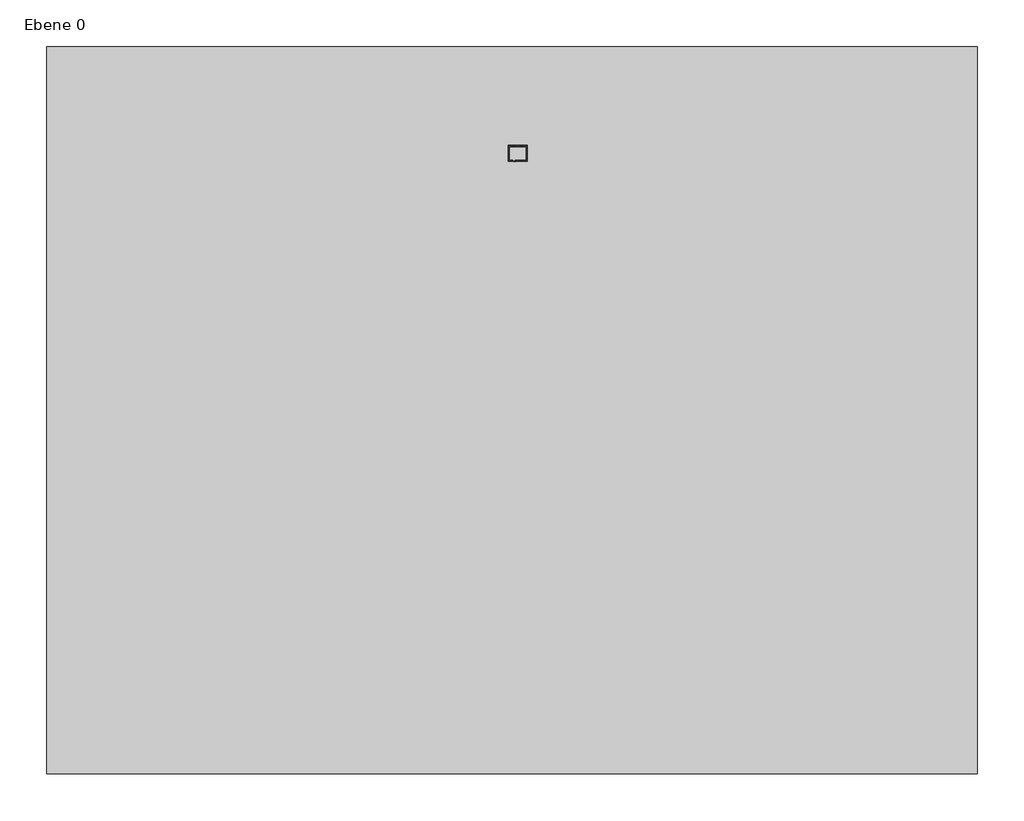
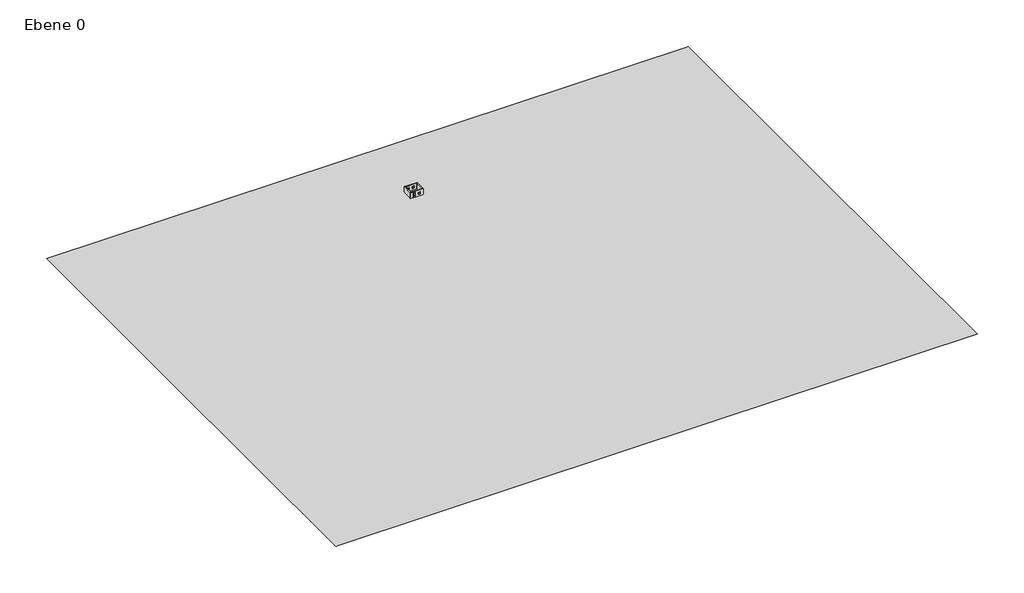
# One storey: 4 walls, 3 windows, 2 proxies, 1 door.
"""IFC4 building model written with IfcOpenShell, lengths in millimetres."""

import ifcopenshell
import ifcopenshell.guid

model = None  # the IFC model being written
_history = None  # IfcOwnerHistory: only IFC2X3 demands one
_inside = {}  # id of a spatial element -> (the spatial element, [elements in it])
_under = {}  # id of a project, library or spatial element -> (it, [spatial elements below it])
_declared = {}  # id of a project -> (the project, [libraries it declares])
_typed = {}  # id of a type object -> (the type object, [elements of that type])
_made_of = {}  # id of a material, layer set ... -> (it, [elements and type objects made of it])


def new_model(schema):
    """Start an empty IFC model of exactly this schema.

    Asked for "IFC4X3", IfcOpenShell would pick the latest addendum, in which some entities
    have other attributes; the version numbers below select the first issue.
    IFC2X3 requires an IfcOwnerHistory on every rooted entity: one is made here for all.
    """
    global model, _history
    if schema == "IFC4X3":
        model = ifcopenshell.file(schema_version=(4, 3, 0, 0))
    else:
        model = ifcopenshell.file(schema=schema)
    _inside.clear()
    _under.clear()
    _declared.clear()
    _typed.clear()
    _made_of.clear()
    _history = None
    if model.schema == "IFC2X3":
        org = make("IfcOrganization", Name="unknown")
        user = make(
            "IfcPersonAndOrganization",
            ThePerson=make("IfcPerson", FamilyName="unknown"),
            TheOrganization=org,
        )
        app = make(
            "IfcApplication",
            ApplicationDeveloper=org,
            Version="unknown",
            ApplicationFullName="unknown",
            ApplicationIdentifier="unknown",
        )
        _history = make(
            "IfcOwnerHistory",
            OwningUser=user,
            OwningApplication=app,
            ChangeAction="ADDED",
            CreationDate=0,
        )
    return model


def make(cls, **values):
    """One entity of the class cls with the attributes given. An attribute that is None is left unset."""
    return model.create_entity(
        cls, **{name: value for name, value in values.items() if value is not None}
    )


def rooted(cls, **values):
    """An entity with a GlobalId (a new one), such as an element, a storey or a relation."""
    return make(cls, GlobalId=ifcopenshell.guid.new(), OwnerHistory=_history, **values)


def si_unit(unit_type, name, prefix=None):
    """IfcSIUnit, for example si_unit("LENGTHUNIT", "METRE", prefix="MILLI")."""
    return make("IfcSIUnit", UnitType=unit_type, Prefix=prefix, Name=name)


def assignment(units):
    """IfcUnitAssignment: the units of a project."""
    return None if units is None else make("IfcUnitAssignment", Units=units)


def point(xyz):
    """IfcCartesianPoint."""
    return None if xyz is None else make("IfcCartesianPoint", Coordinates=xyz)


def direction(xyz):
    """IfcDirection."""
    return None if xyz is None else make("IfcDirection", DirectionRatios=xyz)


def frame(location, z_axis=None, x_axis=None):
    """IfcAxis2Placement3D, a coordinate frame: its origin and axes. An axis left out is left unset."""
    return make(
        "IfcAxis2Placement3D",
        Location=point(location),
        Axis=direction(z_axis),
        RefDirection=direction(x_axis),
    )


def frame_2d(location, x_axis=None):
    """IfcAxis2Placement2D, a coordinate frame in the plane: its origin and x axis."""
    return make(
        "IfcAxis2Placement2D", Location=point(location), RefDirection=direction(x_axis)
    )


def origin():
    """The frame at (0, 0, 0) with its axes left unset."""
    return frame((0.0, 0.0, 0.0))


def origin_with_axes():
    """The frame at (0, 0, 0) with the z axis (0, 0, 1) and the x axis (1, 0, 0) written out."""
    return frame((0.0, 0.0, 0.0), z_axis=(0.0, 0.0, 1.0), x_axis=(1.0, 0.0, 0.0))


def place(relative_to, where):
    """IfcLocalPlacement: puts the frame where relative to a parent placement (None: the world)."""
    return make(
        "IfcLocalPlacement", PlacementRelTo=relative_to, RelativePlacement=where
    )


def context(
    kind, dimensions, precision=None, world=None, true_north=None, identifier=None
):
    """IfcGeometricRepresentationContext, for example the 3D "Model" context."""
    return make(
        "IfcGeometricRepresentationContext",
        ContextIdentifier=identifier,
        ContextType=kind,
        CoordinateSpaceDimension=dimensions,
        Precision=precision,
        WorldCoordinateSystem=world,
        TrueNorth=true_north,
    )


def project(units=None, contexts=None):
    """IfcProject with its units and contexts."""
    return rooted(
        "IfcProject",
        Name="project",
        RepresentationContexts=contexts,
        UnitsInContext=assignment(units),
    )


def spatial(cls, under=None, at=None, **own):
    """A site, building, storey or space (cls), placed at a placement, below another one or the project."""
    s = rooted(cls, ObjectPlacement=at, **own)
    if under is not None:
        _under.setdefault(under.id(), (under, []))[1].append(s)
    return s


def polyline(points):
    """IfcPolyline through the points."""
    return make("IfcPolyline", Points=[point(p) for p in points])


def point_list(points):
    """IfcCartesianPointList2D or 3D."""
    cls = (
        "IfcCartesianPointList2D" if len(points[0]) == 2 else "IfcCartesianPointList3D"
    )
    return make(cls, CoordList=points)


def circle_curve(where, radius):
    """IfcCircle in the frame where."""
    return make("IfcCircle", Position=where, Radius=radius)


def ellipse_curve(where, semi_axis1, semi_axis2):
    """IfcEllipse in the frame where."""
    return make(
        "IfcEllipse", Position=where, SemiAxis1=semi_axis1, SemiAxis2=semi_axis2
    )


def trimmed(basis, trim1, trim2, sense, master):
    """IfcTrimmedCurve: the piece of a basis curve between two trims."""
    return make(
        "IfcTrimmedCurve",
        BasisCurve=basis,
        Trim1=trim1,
        Trim2=trim2,
        SenseAgreement=sense,
        MasterRepresentation=master,
    )


def segment(curve, same_sense, transition):
    """IfcCompositeCurveSegment."""
    return make(
        "IfcCompositeCurveSegment",
        Transition=transition,
        SameSense=same_sense,
        ParentCurve=curve,
    )


def composite_curve(segments, self_intersect=None):
    """IfcCompositeCurve: segments joined end to end."""
    return make("IfcCompositeCurve", Segments=segments, SelfIntersect=self_intersect)


def outline(outer, holes=None, kind="AREA"):
    """IfcArbitraryClosedProfileDef: a profile drawn as a closed curve; with holes, ...WithVoids."""
    if holes is None:
        return make("IfcArbitraryClosedProfileDef", ProfileType=kind, OuterCurve=outer)
    return make(
        "IfcArbitraryProfileDefWithVoids",
        ProfileType=kind,
        OuterCurve=outer,
        InnerCurves=holes,
    )


def extrude(swept, where, along, depth):
    """IfcExtrudedAreaSolid: the profile swept, set in the frame where, extruded along a direction by depth."""
    return make(
        "IfcExtrudedAreaSolid",
        SweptArea=swept,
        Position=where,
        ExtrudedDirection=direction(along),
        Depth=depth,
    )


def faces_of(points, faces, orient=None, outer=None):
    """IfcFace entities. A face is a list of loops; a loop is a list of indices into points, from 0.

    orient and outer hold one flag for each loop. By default every Orientation is true, the
    first loop of a face is its IfcFaceOuterBound and the others are IfcFaceBound.
    """
    made = []
    for i, loops in enumerate(faces):
        bounds = []
        for j, loop in enumerate(loops):
            is_outer = j == 0 if outer is None else outer[i][j]
            bounds.append(
                make(
                    "IfcFaceOuterBound" if is_outer else "IfcFaceBound",
                    Bound=make("IfcPolyLoop", Polygon=[points[k] for k in loop]),
                    Orientation=True if orient is None else orient[i][j],
                )
            )
        made.append(make("IfcFace", Bounds=bounds))
    return made


def faceted_brep(points, faces, orient=None, outer=None, voids=None):
    """IfcFacetedBrep: a solid bounded by flat faces; with voids (closed shells), ...WithVoids."""
    shared = [point(p) for p in points]
    hull = make("IfcClosedShell", CfsFaces=faces_of(shared, faces, orient, outer))
    if voids is None:
        return make("IfcFacetedBrep", Outer=hull)
    return make(
        "IfcFacetedBrepWithVoids",
        Outer=hull,
        Voids=[
            make(cls, CfsFaces=faces_of(shared, fs, o, b)) for cls, fs, o, b in voids
        ],
    )


def triangles(points, corners, closed=None, point_numbers=None):
    """IfcTriangulatedFaceSet: each triangle names its three corners, points numbered from 1."""
    return make(
        "IfcTriangulatedFaceSet",
        Coordinates=point_list(points),
        Closed=closed,
        CoordIndex=corners,
        PnIndex=point_numbers,
    )


def shape(context_of_items, identifier, shape_type, items):
    """IfcShapeRepresentation: the items that make up one representation, for example the "Body"."""
    return make(
        "IfcShapeRepresentation",
        ContextOfItems=context_of_items,
        RepresentationIdentifier=identifier,
        RepresentationType=shape_type,
        Items=items,
    )


def source(mapping_origin, context_of_items, identifier, shape_type, items):
    """IfcRepresentationMap: a shape defined once, which mapped items show again and again."""
    return make(
        "IfcRepresentationMap",
        MappingOrigin=mapping_origin,
        MappedRepresentation=shape(context_of_items, identifier, shape_type, items),
    )


def transform(
    local_origin,
    x_axis=None,
    y_axis=None,
    z_axis=None,
    scale=None,
    scale2=None,
    scale3=None,
    uniform=True,
):
    """IfcCartesianTransformationOperator3D, or its non-uniform kind. x_axis, y_axis, z_axis: its Axis1, 2, 3."""
    if uniform:
        return make(
            "IfcCartesianTransformationOperator3D",
            Axis1=direction(x_axis),
            Axis2=direction(y_axis),
            LocalOrigin=point(local_origin),
            Scale=scale,
            Axis3=direction(z_axis),
        )
    return make(
        "IfcCartesianTransformationOperator3DnonUniform",
        Axis1=direction(x_axis),
        Axis2=direction(y_axis),
        LocalOrigin=point(local_origin),
        Scale=scale,
        Axis3=direction(z_axis),
        Scale2=scale2,
        Scale3=scale3,
    )


def mapped(mapping_source, mapping_target):
    """IfcMappedItem: shows the shape of a source again, moved by a transform."""
    return make(
        "IfcMappedItem", MappingSource=mapping_source, MappingTarget=mapping_target
    )


def made_of(thing, what):
    """Note that an element or type object is made of a material, layer set ...; save() writes the relation."""
    if what is not None:
        _made_of.setdefault(what.id(), (what, []))[1].append(thing)
    return thing


def element(
    cls,
    number,
    at=None,
    inside=None,
    cuts=None,
    type_object=None,
    material=None,
    context=None,
    identifier="Body",
    shape_type=None,
    held_by="IfcProductDefinitionShape",
    body=None,
    shapes=None,
    **own,
):
    """One element of the class cls, such as IfcWall. Its Tag is "e" and its number.

    at: its placement. inside: the storey or other place that contains it. cuts: it is an
    opening in that element (IfcRelVoidsElement). A single representation is given by context,
    identifier, shape_type and body (its items); several are given by shapes. held_by: the class
    of the entity that holds the representations. save() writes the other relations.
    """
    e = rooted(cls, Tag="e%d" % number, ObjectPlacement=at, **own)
    if body is not None:
        shapes = [shape(context, identifier, shape_type, body)]
    if shapes is not None:
        e.Representation = make(held_by, Representations=shapes)
    if inside is not None:
        _inside.setdefault(inside.id(), (inside, []))[1].append(e)
    if cuts is not None:
        rooted(
            "IfcRelVoidsElement", RelatingBuildingElement=cuts, RelatedOpeningElement=e
        )
    if type_object is not None:
        _typed.setdefault(type_object.id(), (type_object, []))[1].append(e)
    return made_of(e, material)


def aggregate(whole, parts):
    """IfcRelAggregates: a whole, such as a stair, and the parts it consists of."""
    return rooted("IfcRelAggregates", RelatingObject=whole, RelatedObjects=parts)


def save(model, path):
    """Write the relations noted so far, then the file.

    IfcRelAggregates (storeys below a building ...), IfcRelContainedInSpatialStructure (elements
    in a storey), IfcRelDefinesByType, IfcRelAssociatesMaterial and IfcRelDeclares: one each for
    every whole, place, type object, material and project.
    """
    for whole, parts in _under.values():
        aggregate(whole, parts)
    for where, things in _inside.values():
        rooted(
            "IfcRelContainedInSpatialStructure",
            RelatedElements=things,
            RelatingStructure=where,
        )
    for kind, things in _typed.values():
        rooted("IfcRelDefinesByType", RelatedObjects=things, RelatingType=kind)
    for what, things in _made_of.values():
        rooted("IfcRelAssociatesMaterial", RelatedObjects=things, RelatingMaterial=what)
    for by, libraries in _declared.values():
        rooted("IfcRelDeclares", RelatingContext=by, RelatedDefinitions=libraries)
    model.write(path)


def plane_surface(at):
    """IfcPlane: the flat surface through the origin of the frame at, square to its z axis."""
    return make("IfcPlane", Position=at)


def cylinder_surface(at, radius):
    """IfcCylindricalSurface: all points at the distance radius from the z axis of the frame at."""
    return make("IfcCylindricalSurface", Position=at, Radius=radius)


def advanced_brep(points, edges, surfaces, faces):
    """IfcAdvancedBrep: a solid bounded by faces that lie on surfaces and meet in shared edges.

    An edge is (start, end): straight between two places in points (the first is 0);
    or (start, end, curve); or (start, end, curve, False) where it runs against its curve.
    A face is (place in surfaces, loops), or (place, loops, False) where it looks against
    its surface's normal. A loop lists edges by number (the first is 1), with a minus sign
    where the edge is run from its end to its start. The first loop is the outer one.
    """
    corners = [point(p) for p in points]
    vertices = [make("IfcVertexPoint", VertexGeometry=c) for c in corners]
    made = []
    for start, end, *more in edges:
        made.append(
            make(
                "IfcEdgeCurve",
                EdgeStart=vertices[start],
                EdgeEnd=vertices[end],
                EdgeGeometry=more[0] if more else make("IfcPolyline", Points=[corners[start], corners[end]]),
                SameSense=more[1] if len(more) > 1 else True,
            )
        )
    hull = []
    for where, loops, *sense in faces:
        bounds = []
        for j, loop in enumerate(loops):
            ring = [make("IfcOrientedEdge", EdgeElement=made[abs(k) - 1], Orientation=k > 0) for k in loop]
            bounds.append(
                make(
                    "IfcFaceOuterBound" if j == 0 else "IfcFaceBound",
                    Bound=make("IfcEdgeLoop", EdgeList=ring),
                    Orientation=True,
                )
            )
        hull.append(make("IfcAdvancedFace", Bounds=bounds, FaceSurface=surfaces[where], SameSense=sense[0] if sense else True))
    return make("IfcAdvancedBrep", Outer=make("IfcClosedShell", CfsFaces=hull))


def door_88_5_x_2_26_80f06d6c(model_context):
    return source(origin(), model_context, "Body", "SolidModel", [
        advanced_brep(
        [(-352.5, 169.4346141, 1000.0), (-332.5, 169.4346141, 1000.0), (-352.5, 99.4346141, 1000.0), (-332.5, 119.4346141, 1000.0), (-222.5, 99.4346141, 1000.0), (-222.5, 119.4346141, 1000.0)],
        [
            (0, 1, circle_curve(frame((-342.5, 169.4346141, 1000.0), z_axis=(0.0, 1.0, 0.0), x_axis=(1.0, 0.0, 0.0)), 10.0)),
            (1, 0, circle_curve(frame((-342.5, 169.4346141, 1000.0), z_axis=(0.0, 1.0, 0.0), x_axis=(1.0, 0.0, 0.0)), 10.0)),
            (0, 2),
            (2, 3, ellipse_curve(frame((-342.5, 109.4346141, 1000.0), z_axis=(-0.7071067811865385, 0.7071067811865565, 0.0), x_axis=(0.7071067811865563, 0.7071067811865386, 0.0)), 14.1421356, 10.0)),
            (3, 1),
            (3, 2, ellipse_curve(frame((-342.5, 109.4346141, 1000.0), z_axis=(-0.7071067811865385, 0.7071067811865565, 0.0), x_axis=(0.7071067811865563, 0.7071067811865386, 0.0)), 14.1421356, 10.0)),
            (4, 5, circle_curve(frame((-222.5, 109.4346141, 1000.0), z_axis=(1.0, 0.0, 0.0), x_axis=(0.0, 1.0, 0.0)), 10.0)),
            (5, 4, circle_curve(frame((-222.5, 109.4346141, 1000.0), z_axis=(1.0, 0.0, 0.0), x_axis=(0.0, 1.0, 0.0)), 10.0)),
            (2, 4),
            (5, 3),
        ],
        [
            plane_surface(frame((-342.5, 169.4346141, -287.7526403), z_axis=(0.0, 1.0, 0.0), x_axis=(0.0, 0.0, 1.0))),
            cylinder_surface(frame((-342.5, 169.4346141, 1000.0), z_axis=(0.0, 1.0, 0.0), x_axis=(1.0, 0.0, 0.0)), 10.0),
            plane_surface(frame((-222.5, 109.4346141, -287.7526403), z_axis=(1.0, 0.0, 0.0), x_axis=(0.0, 0.0, 1.0))),
            cylinder_surface(frame((-342.5, 109.4346141, 1000.0), z_axis=(-1.0, 0.0, 0.0), x_axis=(0.0, 1.0, 0.0)), 10.0),
        ],
        [
            (0, [[1, 2]]),
            (1, [[-1, 3, 4, 5]]),
            (1, [[-2, -5, 6, -3]]),
            (2, [[7, 8]]),
            (3, [[-4, 9, -8, 10]]),
            (3, [[-6, -10, -7, -9]]),
        ],
    ),
        advanced_brep(
        [(-332.5, 229.4346141, 1000.0), (-352.5, 229.4346141, 1000.0), (-332.5, 259.4346141, 1000.0), (-352.5, 279.4346141, 1000.0), (-222.5, 259.4346141, 1000.0), (-222.5, 279.4346141, 1000.0)],
        [
            (0, 1, circle_curve(frame((-342.5, 229.4346141, 1000.0), z_axis=(0.0, -1.0, 0.0), x_axis=(-1.0, 0.0, 0.0)), 10.0)),
            (1, 0, circle_curve(frame((-342.5, 229.4346141, 1000.0), z_axis=(0.0, -1.0, 0.0), x_axis=(-1.0, 0.0, 0.0)), 10.0)),
            (0, 2),
            (2, 3, ellipse_curve(frame((-342.5, 269.4346141, 1000.0), z_axis=(-0.7071067811865475, -0.7071067811865475, 0.0), x_axis=(0.7071067811865474, -0.7071067811865476, 0.0)), 14.1421356, 10.0)),
            (3, 1),
            (3, 2, ellipse_curve(frame((-342.5, 269.4346141, 1000.0), z_axis=(-0.7071067811865475, -0.7071067811865475, 0.0), x_axis=(0.7071067811865474, -0.7071067811865476, 0.0)), 14.1421356, 10.0)),
            (4, 5, circle_curve(frame((-222.5, 269.4346141, 1000.0), z_axis=(1.0, 0.0, 0.0), x_axis=(0.0, 1.0, 0.0)), 10.0)),
            (5, 4, circle_curve(frame((-222.5, 269.4346141, 1000.0), z_axis=(1.0, 0.0, 0.0), x_axis=(0.0, 1.0, 0.0)), 10.0)),
            (2, 4),
            (5, 3),
        ],
        [
            plane_surface(frame((-342.5, 229.4346141, -287.7526403), z_axis=(0.0, -1.0, 0.0), x_axis=(0.0, 0.0, 1.0))),
            cylinder_surface(frame((-342.5, 229.4346141, 1000.0), z_axis=(0.0, -1.0, 0.0), x_axis=(-1.0, 0.0, 0.0)), 10.0),
            plane_surface(frame((-222.5, 269.4346141, -287.7526403), z_axis=(1.0, 0.0, 0.0), x_axis=(0.0, 0.0, 1.0))),
            cylinder_surface(frame((-342.5, 269.4346141, 1000.0), z_axis=(-1.0, 0.0, 0.0), x_axis=(0.0, 1.0, 0.0)), 10.0),
        ],
        [
            (0, [[1, 2]]),
            (1, [[-1, 3, 4, 5]]),
            (1, [[-2, -5, 6, -3]]),
            (2, [[7, 8]]),
            (3, [[-4, 9, -8, 10]]),
            (3, [[-6, -10, -7, -9]]),
        ],
    ),
        extrude(outline(composite_curve([segment(trimmed(circle_curve(frame_2d((1000.0, -342.5)), 20.0), [point((1000.0, -362.5))], [point((1000.0, -322.5))], False, "CARTESIAN"), True, "CONTINUOUS"), segment(trimmed(circle_curve(frame_2d((1000.0, -342.5)), 20.0), [point((1000.0, -322.5))], [point((1000.0, -362.5))], False, "CARTESIAN"), True, "CONTINUOUS")], self_intersect=False)), frame((0.0, 159.4346141, 0.0), z_axis=(0.0, 1.0, 0.0), x_axis=(0.0, 0.0, 1.0)), (0.0, 0.0, 1.0), 10.0),
        extrude(outline(composite_curve([segment(trimmed(circle_curve(frame_2d((1000.0, -342.5)), 20.0), [point((1000.0, -362.5))], [point((1000.0, -322.5))], False, "CARTESIAN"), True, "CONTINUOUS"), segment(trimmed(circle_curve(frame_2d((1000.0, -342.5)), 20.0), [point((1000.0, -322.5))], [point((1000.0, -362.5))], False, "CARTESIAN"), True, "CONTINUOUS")], self_intersect=False)), frame((0.0, 219.4346141, 0.0), z_axis=(0.0, 1.0, 0.0), x_axis=(0.0, 0.0, 1.0)), (0.0, 0.0, 1.0), 10.0),
        extrude(outline(polyline([(432.5, 194.4346141), (-432.5, 194.4346141), (-432.5, 219.4346141), (432.5, 219.4346141), (432.5, 194.4346141)])), frame((0.0, 0.0, 100.0), z_axis=(0.0, 0.0, 1.0), x_axis=(1.0, 0.0, 0.0)), (0.0, 0.0, 1.0), 2250.0),
        faceted_brep([(466.9603207, -180.5653859, 100.0), (417.5, -180.5653859, 100.0), (417.5, 194.4346141, 100.0), (432.5, 194.4346141, 100.0), (432.5, 219.4346141, 100.0), (466.9603207, 219.4346141, 100.0), (466.9603207, 194.4346141, 100.0), (461.9603207, 194.4346141, 100.0), (461.9603207, 214.4346141, 100.0), (437.5, 214.4346141, 100.0), (437.5, 189.4346141, 100.0), (422.5, 189.4346141, 100.0), (422.5, -175.5653859, 100.0), (461.9603207, -175.5653859, 100.0), (461.9603207, -165.5653859, 100.0), (466.9603207, -165.5653859, 100.0), (466.9603207, -180.5653859, 2384.4603207), (-466.9603207, -180.5653859, 2384.4603207), (-466.9603207, -180.5653859, 100.0), (-417.5, -180.5653859, 100.0), (-417.5, -180.5653859, 2335.0), (417.5, -180.5653859, 2335.0), (417.5, 194.4346141, 2335.0), (-417.5, 194.4346141, 2335.0), (-417.5, 194.4346141, 100.0), (-432.5, 194.4346141, 100.0), (-432.5, 194.4346141, 2350.0), (432.5, 194.4346141, 2350.0), (432.5, 219.4346141, 2350.0), (-432.5, 219.4346141, 2350.0), (-432.5, 219.4346141, 100.0), (-466.9603207, 219.4346141, 100.0), (-466.9603207, 219.4346141, 2384.4603207), (466.9603207, 219.4346141, 2384.4603207), (466.9603207, 194.4346141, 2384.4603207), (-466.9603207, 194.4346141, 2384.4603207), (-466.9603207, 194.4346141, 100.0), (-461.9603207, 194.4346141, 100.0), (-461.9603207, 194.4346141, 2379.4603207), (461.9603207, 194.4346141, 2379.4603207), (461.9603207, 214.4346141, 2379.4603207), (-461.9603207, 214.4346141, 2379.4603207), (-461.9603207, 214.4346141, 100.0), (-437.5, 214.4346141, 100.0), (-437.5, 214.4346141, 2355.0), (437.5, 214.4346141, 2355.0), (437.5, 189.4346141, 2355.0), (-437.5, 189.4346141, 2355.0), (-437.5, 189.4346141, 100.0), (-422.5, 189.4346141, 100.0), (-422.5, 189.4346141, 2340.0), (422.5, 189.4346141, 2340.0), (422.5, -175.5653859, 2340.0), (-422.5, -175.5653859, 2340.0), (-422.5, -175.5653859, 100.0), (-461.9603207, -175.5653859, 100.0), (-461.9603207, -175.5653859, 2379.4603207), (461.9603207, -175.5653859, 2379.4603207), (461.9603207, -165.5653859, 2379.4603207), (-461.9603207, -165.5653859, 2379.4603207), (-461.9603207, -165.5653859, 100.0), (-466.9603207, -165.5653859, 100.0), (-466.9603207, -165.5653859, 2384.4603207), (466.9603207, -165.5653859, 2384.4603207)], [[[0, 1, 2, 3, 4, 5, 6, 7, 8, 9, 10, 11, 12, 13, 14, 15]], [[1, 0, 16, 17, 18, 19, 20, 21]], [[2, 1, 21, 22]], [[3, 2, 22, 23, 24, 25, 26, 27]], [[4, 3, 27, 28]], [[5, 4, 28, 29, 30, 31, 32, 33]], [[6, 5, 33, 34]], [[7, 6, 34, 35, 36, 37, 38, 39]], [[8, 7, 39, 40]], [[9, 8, 40, 41, 42, 43, 44, 45]], [[10, 9, 45, 46]], [[11, 10, 46, 47, 48, 49, 50, 51]], [[12, 11, 51, 52]], [[13, 12, 52, 53, 54, 55, 56, 57]], [[14, 13, 57, 58]], [[15, 14, 58, 59, 60, 61, 62, 63]], [[0, 15, 63, 16]], [[17, 62, 61, 18]], [[18, 61, 60, 55, 54, 49, 48, 43, 42, 37, 36, 31, 30, 25, 24, 19]], [[23, 20, 19, 24]], [[29, 26, 25, 30]], [[35, 32, 31, 36]], [[41, 38, 37, 42]], [[47, 44, 43, 48]], [[53, 50, 49, 54]], [[59, 56, 55, 60]], [[22, 21, 20, 23]], [[28, 27, 26, 29]], [[34, 33, 32, 35]], [[40, 39, 38, 41]], [[46, 45, 44, 47]], [[52, 51, 50, 53]], [[58, 57, 56, 59]], [[16, 63, 62, 17]]]),
    ])


def fenster_1_flg_variabel_fenster_1_flg_variabel_3_8a378bad(model_context):
    return source(origin(), model_context, "Body", "SolidModel", [
        extrude(outline(polyline([(2010.0, 505.0), (2010.0, -505.0), (1000.0, -505.0), (1000.0, 505.0), (2010.0, 505.0)]), holes=[polyline([(1930.0, 445.0), (1080.0, 445.0), (1080.0, -445.0), (1930.0, -445.0), (1930.0, 445.0)])]), frame((0.0, 40.0, 0.0), z_axis=(0.0, 1.0, 0.0), x_axis=(0.0, 0.0, 1.0)), (0.0, 0.0, 1.0), 60.0),
        faceted_brep([(475.0, 40.0, 1960.0), (475.0, 10.0, 1960.0), (475.0, 10.0, 1050.0), (475.0, 40.0, 1050.0), (-475.0, 10.0, 1960.0), (-475.0, 10.0, 1050.0), (415.0, 10.0, 1110.0), (-415.0, 10.0, 1110.0), (-415.0, 10.0, 1900.0), (415.0, 10.0, 1900.0), (-475.0, 40.0, 1050.0), (-475.0, 40.0, 1960.0), (445.0, 40.0, 1930.0), (-445.0, 40.0, 1930.0), (-445.0, 40.0, 1080.0), (445.0, 40.0, 1080.0), (445.0, 70.0, 1930.0), (445.0, 70.0, 1080.0), (-445.0, 70.0, 1080.0), (-445.0, 70.0, 1930.0), (415.0, 70.0, 1900.0), (-415.0, 70.0, 1900.0), (-415.0, 70.0, 1110.0), (415.0, 70.0, 1110.0)], [[[0, 1, 2, 3]], [[1, 4, 5, 2], [6, 7, 8, 9]], [[3, 2, 5, 10]], [[3, 10, 11, 0], [12, 13, 14, 15]], [[16, 12, 15, 17]], [[17, 15, 14, 18]], [[17, 18, 19, 16], [20, 21, 22, 23]], [[9, 20, 23, 6]], [[6, 23, 22, 7]], [[10, 5, 4, 11]], [[18, 14, 13, 19]], [[7, 22, 21, 8]], [[11, 4, 1, 0]], [[19, 13, 12, 16]], [[8, 21, 20, 9]]]),
        extrude(outline(polyline([(-505.0, -210.0), (-505.0, 40.0), (505.0, 40.0), (505.0, -210.0), (-505.0, -210.0)])), frame((0.0, 0.0, 1005.0), z_axis=(0.0, 0.0, 1.0), x_axis=(1.0, 0.0, 0.0)), (0.0, 0.0, 1.0), 15.0),
        extrude(outline(polyline([(110.0221543, 1020.0), (210.0, 1000.0), (210.0, 990.0), (208.0, 990.0), (208.0, 998.3604634), (109.8240723, 1018.0), (100.0, 1018.0), (100.0, 1020.0), (110.0221543, 1020.0)])), frame((-505.0, 0.0, 0.0), z_axis=(1.0, 0.0, 0.0), x_axis=(0.0, 1.0, 0.0)), (0.0, 0.0, 1.0), 1010.0),
        extrude(outline(polyline([(415.0, 25.0), (-415.0, 25.0), (-415.0, 55.0), (415.0, 55.0), (415.0, 25.0)])), frame((0.0, 0.0, 1110.0), z_axis=(0.0, 0.0, 1.0), x_axis=(1.0, 0.0, 0.0)), (0.0, 0.0, 1.0), 790.0),
    ])


model = new_model("IFC4")

# Units and contexts
model_context = context("Model", 3, world=origin())
ifc_project = project(units=[si_unit("LENGTHUNIT", "METRE", prefix="MILLI")], contexts=[model_context])

# Site, building, storey
site = spatial("IfcSite", under=ifc_project)
building = spatial("IfcBuilding", under=site)
storey = spatial("IfcBuildingStorey", under=building, Name="Ebene 0", Elevation=0.0)

# Proxies
placement = place(None, origin())
element("IfcBuildingElementProxy", 1, Name="Building Element Proxy", at=placement, inside=storey, context=model_context, shape_type="Tessellation", body=[
    triangles([(-160331.1996094, -65742.4011108, 0.0), (-160331.1996094, -208151.4062988, 0.0), (23848.9001038, -208151.4062988, 0.0), (12197.4996643, -199419.9020508, 0.0), (-5694.3001007, -186011.6041992, 0.0), (-25481.9004272, -171004.4085938, 0.0), (-41498.6018555, -156049.302832, 0.0), (-55953.3009521, -142550.7035156, 0.0), (-81517.601001, -122551.5986572, 0.0), (-90344.9970703, -115644.9969727, 0.0), (-95745.3, -111898.3977539, 0.0), (-139582.1033203, -81515.7034424, 0.0), (154493.6024414, -208151.4062988, 0.0), (154493.6024414, -146509.2990967, 0.0), (152327.2974609, -183778.6986328, 0.0), (151970.2029785, -191029.9025391, 0.0), (131234.6407471, -189976.3854492, 0.0), (128010.9956543, -189812.6000977, 0.0), (103567.5016113, -191451.7000488, 0.0), (73532.4977051, -193637.296875, 0.0), (59545.7979492, -197106.1083984, 0.0), (45621.6990234, -200561.3021484, 0.0), (35421.8006836, -204117.6060059, 0.0), (25840.2994812, -207458.2951172, 0.0), (154493.6024414, 37859.0007568, 0.0), (-45179.0004639, 37859.0007568, 0.0), (-20995.999823, -3482.9999016, 0.0), (-20185.0004883, -4870.0001244, 0.0), (-16502.099707, -11166.2998169, 0.0), (-5863.3002502, -5298.2998535, 0.0), (4055.6001251, 223.0999905, 0.0), (14232.299881, 5042.7997513, 0.0), (20896.8988953, 7816.7002029, 0.0), (23379.4008545, 2726.9001228, 0.0), (32183.900647, -15324.6994812, 0.0), (35127.4000488, -15951.6995819, 0.0), (51396.7000122, -19416.9996918, 0.0), (71552.5022827, -34777.0005066, 0.0), (89162.3994873, -48196.3000122, 0.0), (97424.6021484, -54516.300293, 0.0), (103453.3969482, -59668.902063, 0.0), (125381.6956787, -79503.9006592, 0.0), (138980.4005127, -76672.5013916, 0.0), (142103.1959473, -85544.0994141, 0.0), (152666.9046387, -116932.3044434, 0.0), (-160331.1996094, 37859.0007568, 0.0), (-157617.8024414, -59206.6000488, 0.0), (-156348.2055176, -56148.4006714, 0.0), (-133528.5007324, -3798.9000961, 0.0), (-116015.0022949, -11087.9999451, 0.0), (-107594.0000244, -6686.0000336, 0.0), (-104346.1517578, -5888.8399704, 0.0), (-103918.9964355, -5783.9998581, 0.0), (-102571.999585, -5452.9997131, 0.0), (-102346.0040771, -5318.9997528, 0.0), (-100888.0000488, -4452.9999962, 0.0), (-98390.0036865, -3171.9999893, 0.0), (-95145.0017578, -1507.0000202, 0.0), (-87760.0013672, 3877.9999191, 0.0), (-87175.9998047, 4304.0000793, 0.0), (-73718.9979492, 7734.0000183, 0.0), (-75124.0005615, 10122.9995453, 0.0), (-76451.9985718, 12378.0002747, 0.0), (-73623.9990967, 14575.9998322, 0.0), (-67567.0013672, 20473.9991272, 0.0), (-64063.0012939, 24429.9995178, 0.0), (-58507.0008911, 30701.0004639, 0.0), (-58376.9995239, 30747.9999207, 0.0)], [[1, 2, 12], [47, 12, 48], [12, 47, 1], [50, 12, 11], [46, 1, 47], [48, 50, 49], [48, 12, 50], [56, 51, 52], [52, 51, 50], [50, 53, 52], [50, 51, 49], [12, 2, 11], [46, 47, 48], [10, 29, 11], [9, 2, 8], [9, 29, 10], [8, 2, 7], [10, 2, 9], [9, 8, 29], [53, 54, 55], [53, 50, 54], [57, 55, 11], [11, 55, 54], [11, 2, 10], [58, 11, 29], [50, 11, 54], [52, 53, 56], [35, 8, 7], [7, 2, 6], [2, 5, 6], [55, 56, 53], [51, 57, 49], [57, 51, 56], [49, 57, 59], [57, 11, 58], [55, 57, 56], [59, 57, 58], [46, 59, 60], [59, 46, 49], [60, 63, 46], [63, 60, 62], [59, 61, 60], [46, 63, 65], [58, 61, 59], [49, 46, 48], [62, 61, 64], [61, 62, 60], [65, 61, 27], [61, 65, 64], [27, 61, 28], [62, 64, 63], [66, 46, 65], [65, 27, 66], [67, 68, 26], [68, 67, 66], [68, 66, 27], [67, 26, 46], [26, 68, 27], [67, 46, 66], [27, 31, 26], [63, 64, 65], [58, 29, 61], [7, 6, 38], [4, 3, 24], [24, 13, 23], [4, 24, 23], [21, 22, 23], [21, 23, 13], [4, 23, 22], [4, 22, 5], [4, 5, 2], [5, 21, 39], [13, 20, 21], [22, 21, 5], [20, 40, 21], [24, 3, 13], [3, 4, 2], [18, 13, 17], [13, 18, 19], [16, 13, 15], [13, 16, 17], [19, 20, 13], [17, 16, 15], [19, 18, 14], [42, 19, 45], [45, 19, 14], [14, 15, 13], [45, 14, 25], [18, 17, 14], [17, 15, 14], [44, 45, 25], [19, 42, 20], [44, 42, 45], [28, 29, 30], [28, 61, 29], [30, 35, 31], [35, 30, 29], [35, 29, 8], [30, 31, 27], [32, 26, 31], [32, 31, 34], [37, 33, 34], [34, 33, 32], [31, 35, 34], [33, 26, 32], [34, 35, 36], [28, 30, 27], [25, 40, 41], [39, 38, 6], [42, 43, 41], [43, 42, 44], [40, 39, 21], [25, 41, 43], [37, 25, 33], [37, 36, 38], [38, 39, 25], [36, 35, 7], [25, 39, 40], [38, 25, 37], [38, 36, 7], [37, 34, 36], [43, 44, 25], [41, 40, 20], [20, 42, 41], [33, 25, 26], [39, 6, 5]], closed=False),
])
element("IfcBuildingElementProxy", 2, Name="Building Element Proxy", at=placement, inside=storey, context=model_context, shape_type="Tessellation", body=[
    triangles([(-20995.999823, -3482.9999016, 0.0), (-45179.0004639, 37859.0007568, 0.0), (-58376.9995239, 30747.9999207, 0.0), (-58507.0008911, 30701.0004639, 0.0), (-64063.0012939, 24429.9995178, 0.0), (-67567.0013672, 20473.9991272, 0.0), (-73623.9990967, 14575.9998322, 0.0), (-76451.9985718, 12378.0002747, 0.0), (-75124.0005615, 10122.9995453, 0.0), (-73718.9979492, 7734.0000183, 0.0), (-87175.9998047, 4304.0000793, 0.0), (-87760.0013672, 3877.9999191, 0.0), (-95145.0017578, -1507.0000202, 0.0), (-98390.0036865, -3171.9999893, 0.0), (-100888.0000488, -4452.9999962, 0.0), (-102346.0040771, -5318.9997528, 0.0), (-102571.999585, -5452.9997131, 0.0), (-103918.9964355, -5783.9998581, 0.0), (-104346.1517578, -5888.8399704, 0.0), (-107594.0000244, -6686.0000336, 0.0), (-116015.0022949, -11087.9999451, 0.0), (-133528.5007324, -3798.9000961, 0.0), (-156348.2055176, -56148.4006714, 0.0), (-157617.8024414, -59206.6000488, 0.0), (-160331.1996094, -65742.4011108, 0.0), (-139582.1033203, -81515.7034424, 0.0), (-95745.3, -111898.3977539, 0.0), (-90344.9970703, -115644.9969727, 0.0), (-81517.601001, -122551.5986572, 0.0), (-55953.3009521, -142550.7035156, 0.0), (-41498.6018555, -156049.302832, 0.0), (-25481.9004272, -171004.4085938, 0.0), (-5694.3001007, -186011.6041992, 0.0), (12197.4996643, -199419.9020508, 0.0), (23848.9001038, -208151.4062988, 0.0), (25840.2994812, -207458.2951172, 0.0), (35421.8006836, -204117.6060059, 0.0), (45621.6990234, -200561.3021484, 0.0), (59545.7979492, -197106.1083984, 0.0), (73532.4977051, -193637.296875, 0.0), (103567.5016113, -191451.7000488, 0.0), (128010.9956543, -189812.6000977, 0.0), (131234.6407471, -189976.3854492, 0.0), (151970.2029785, -191029.9025391, 0.0), (152327.2974609, -183778.6986328, 0.0), (154493.6024414, -146509.2990967, 0.0), (152666.9046387, -116932.3044434, 0.0), (142103.1959473, -85544.0994141, 0.0), (138980.4005127, -76672.5013916, 0.0), (125381.6956787, -79503.9006592, 0.0), (103453.3969482, -59668.902063, 0.0), (97424.6021484, -54516.300293, 0.0), (89162.3994873, -48196.3000122, 0.0), (71552.5022827, -34777.0005066, 0.0), (51396.7000122, -19416.9996918, 0.0), (35127.4000488, -15951.6995819, 0.0), (32183.900647, -15324.6994812, 0.0), (23379.4008545, 2726.9001228, 0.0), (20896.8988953, 7816.7002029, 0.0), (14232.299881, 5042.7997513, 0.0), (4055.6001251, 223.0999905, 0.0), (-5863.3002502, -5298.2998535, 0.0), (-16502.099707, -11166.2998169, 0.0), (-20185.0004883, -4870.0001244, 0.0)], [[24, 25, 26], [23, 26, 21], [26, 23, 24], [20, 21, 19], [18, 19, 21], [18, 21, 17], [21, 26, 27], [23, 21, 22], [28, 63, 27], [29, 63, 28], [29, 30, 63], [16, 17, 27], [16, 27, 14], [17, 21, 27], [13, 27, 63], [57, 30, 31], [14, 27, 13], [16, 14, 15], [8, 9, 7], [10, 11, 12], [12, 13, 10], [10, 7, 9], [7, 10, 6], [6, 1, 5], [1, 6, 10], [1, 10, 64], [4, 5, 3], [3, 5, 1], [1, 2, 3], [13, 63, 10], [31, 32, 54], [34, 35, 36], [34, 36, 37], [34, 37, 38], [34, 38, 33], [33, 39, 53], [38, 39, 33], [40, 52, 39], [41, 42, 46], [42, 43, 46], [45, 43, 44], [46, 47, 41], [46, 43, 45], [41, 47, 50], [41, 50, 40], [48, 50, 47], [64, 10, 63], [62, 57, 61], [57, 62, 63], [57, 63, 30], [60, 61, 58], [58, 59, 60], [61, 57, 58], [53, 54, 32], [49, 50, 48], [52, 53, 39], [55, 56, 54], [56, 57, 31], [54, 56, 31], [51, 52, 40], [40, 50, 51], [53, 32, 33]], closed=False),
])

# Door
door_88_5_x_2_26_shape = door_88_5_x_2_26_80f06d6c(model_context)
element("IfcDoor", 3, ObjectType="Drehflügel 1-flg - Stahlzarge : 88.5 x 2.26", at=placement, inside=storey, context=model_context, shape_type="MappedRepresentation", body=[
    mapped(door_88_5_x_2_26_shape, transform((-2223.9979049, -761.1961342, 0.0), x_axis=(-1.0, 0.0, 0.0), y_axis=(0.0, -1.0, 0.0), z_axis=(0.0, 0.0, 1.0))),
])

# Walls
element("IfcWall", 4, ObjectType="MW 24.0 WD 12.0", at=placement, inside=storey, context=model_context, shape_type="Brep", body=[
    faceted_brep([(-3766.4979049, 4044.3692517, 0.0), (1873.5020951, 4044.3692517, 0.0), (1873.5020951, 4044.3692517, 3000.0), (-3766.4979049, 4044.3692517, 3000.0), (673.5020951, 4044.3692517, 1000.0), (-336.4979049, 4044.3692517, 1000.0), (-336.4979049, 4044.3692517, 2010.0), (673.5020951, 4044.3692517, 2010.0), (-1956.4979049, 4044.3692517, 1000.0), (-2966.4979049, 4044.3692517, 1000.0), (-2966.4979049, 4044.3692517, 2010.0), (-1956.4979049, 4044.3692517, 2010.0), (-4126.4979049, 4404.3692517, 0.0), (-4126.4979049, 4404.3692517, 3000.0), (2233.5020951, 4404.3692517, 3000.0), (2233.5020951, 4404.3692517, 0.0), (673.5020951, 4404.3692517, 1000.0), (673.5020951, 4404.3692517, 2010.0), (-336.4979049, 4404.3692517, 2010.0), (-336.4979049, 4404.3692517, 1000.0), (-1956.4979049, 4404.3692517, 1000.0), (-1956.4979049, 4404.3692517, 2010.0), (-2966.4979049, 4404.3692517, 2010.0), (-2966.4979049, 4404.3692517, 1000.0)], [[[0, 1, 2, 3], [4, 5, 6, 7], [8, 9, 10, 11]], [[12, 13, 14, 15], [16, 17, 18, 19], [20, 21, 22, 23]], [[1, 0, 12, 15]], [[3, 2, 14, 13]], [[17, 16, 4, 7]], [[18, 17, 7, 6]], [[19, 18, 6, 5]], [[16, 19, 5, 4]], [[21, 20, 8, 11]], [[22, 21, 11, 10]], [[23, 22, 10, 9]], [[20, 23, 9, 8]], [[0, 3, 13, 12]], [[2, 1, 15, 14]]]),
])
element("IfcWall", 5, ObjectType="MW 24.0 WD 12.0", at=placement, inside=storey, context=model_context, shape_type="SweptSolid", body=[
    extrude(outline(polyline([(1873.5020951, -595.6307483), (1873.5020951, 4044.3692517), (2233.5020951, 4404.3692517), (2233.5020951, -955.6307483), (1873.5020951, -595.6307483)])), origin_with_axes(), (0.0, 0.0, 1.0), 3000.0),
])
element("IfcWall", 6, ObjectType="MW 24.0 WD 12.0", at=placement, inside=storey, context=model_context, shape_type="Brep", body=[
    faceted_brep([(-3766.4979049, -595.6307483, 3000.0), (1873.5020951, -595.6307483, 3000.0), (1873.5020951, -595.6307483, 0.0), (-1781.4979049, -595.6307483, 0.0), (-1781.4979049, -595.6307483, 2360.0), (-2666.4979049, -595.6307483, 2360.0), (-2666.4979049, -595.6307483, 0.0), (-3766.4979049, -595.6307483, 0.0), (-336.4979049, -595.6307483, 1000.0), (673.5020951, -595.6307483, 1000.0), (673.5020951, -595.6307483, 2010.0), (-336.4979049, -595.6307483, 2010.0), (2233.5020951, -955.6307483, 3000.0), (-4126.4979049, -955.6307483, 3000.0), (-4126.4979049, -955.6307483, 0.0), (-2666.4979049, -955.6307483, 0.0), (-2666.4979049, -955.6307483, 2360.0), (-1781.4979049, -955.6307483, 2360.0), (-1781.4979049, -955.6307483, 0.0), (2233.5020951, -955.6307483, 0.0), (-336.4979049, -955.6307483, 1000.0), (-336.4979049, -955.6307483, 2010.0), (673.5020951, -955.6307483, 2010.0), (673.5020951, -955.6307483, 1000.0)], [[[0, 1, 2, 3, 4, 5, 6, 7], [8, 9, 10, 11]], [[12, 13, 14, 15, 16, 17, 18, 19], [20, 21, 22, 23]], [[2, 19, 18, 3]], [[14, 7, 6, 15]], [[1, 0, 13, 12]], [[5, 16, 15, 6]], [[16, 5, 4, 17]], [[17, 4, 3, 18]], [[21, 20, 8, 11]], [[22, 21, 11, 10]], [[23, 22, 10, 9]], [[20, 23, 9, 8]], [[2, 1, 12, 19]], [[0, 7, 14, 13]]]),
])
element("IfcWall", 7, ObjectType="MW 24.0 WD 12.0", at=placement, inside=storey, context=model_context, shape_type="SweptSolid", body=[
    extrude(outline(polyline([(-3766.4979049, 4044.3692517), (-3766.4979049, -595.6307483), (-4126.4979049, -955.6307483), (-4126.4979049, 4404.3692517), (-3766.4979049, 4044.3692517)])), origin_with_axes(), (0.0, 0.0, 1.0), 3000.0),
])

# Windows
fenster_1_flg_variabel_fenster_1_flg_variabel_3_shape = fenster_1_flg_variabel_fenster_1_flg_variabel_3_8a378bad(model_context)
element("IfcWindow", 8, ObjectType="Fenster 1-flg - Variabel : Fenster 1-flg - Variabel 3", at=placement, inside=storey, context=model_context, shape_type="MappedRepresentation", body=[
    mapped(fenster_1_flg_variabel_fenster_1_flg_variabel_3_shape, transform((168.5020951, -775.6307483, 0.0), x_axis=(1.0, 0.0, 0.0), y_axis=(0.0, 1.0, 0.0), z_axis=(0.0, 0.0, 1.0))),
])
element("IfcWindow", 9, ObjectType="Fenster 1-flg - Variabel : Fenster 1-flg - Variabel 3", at=placement, inside=storey, context=model_context, shape_type="MappedRepresentation", body=[
    mapped(fenster_1_flg_variabel_fenster_1_flg_variabel_3_shape, transform((168.5020951, 4224.3692517, 0.0), x_axis=(-1.0, 0.0, 0.0), y_axis=(0.0, -1.0, 0.0), z_axis=(0.0, 0.0, 1.0))),
])
element("IfcWindow", 10, ObjectType="Fenster 1-flg - Variabel : Fenster 1-flg - Variabel 3", at=placement, inside=storey, context=model_context, shape_type="MappedRepresentation", body=[
    mapped(fenster_1_flg_variabel_fenster_1_flg_variabel_3_shape, transform((-2461.4979049, 4224.3692517, 0.0), x_axis=(-1.0, 0.0, 0.0), y_axis=(0.0, -1.0, 0.0), z_axis=(0.0, 0.0, 1.0))),
])

save(model, "model.ifc")

# Revit data of these elements
# Project information
#   Testproperty = "TestpropertyValue"
#   Bezeichnung des Bauvorhabens = "LandBIM Bauvorhaben"
#   Projektausgabedatum = "Projekt Datum"
#   Projektstatus = "Projektstatus"
#   Auftraggeber = "Walter Beispiel"
#   Projektadresse = "Zufallweg 2"
#   Projektname = "Projektname"
#   Projektnummer = "Projektnummer"
#   Verfasser Firma 1 = "Firma 1"
#   Verfasser Firma 2 = "Firma 2"
#   Verfasser PLZ Ort = "PLZ Ort"
#   Verfasser Strasse = "Strasse"
#   Verfasser Telefon = "Telefon"
#   Verfasser Telefax = "Telefax"
#   Verfasser eMail = "E-Mail"
# Type "Drehflügel 1-flg - Stahlzarge : 88.5 x 2.26"
#   Construction Type Id = "MDOOR"
#   Type Mark = "20"
#   Operation = "SingleSwingRight"
#   Keynote = "16.03"
#   Analytic Construction = "Metall"
#   Thermal Resistance (R) = 0.270117 (m²·K)/W
#   Heat Transfer Coefficient (U) = 3.7021 W/(m²·K)
#   Rough Width = 0.885 m
#   Rough Height [instance default] = 2.360 m
#   Höhe Türgriff [instance default] = 0.900 m
#   Height = 2.260 m
#   Fußbodenaufbau [instance default] = 0.100 m
#   Width = 0.885 m
#   Define Thermal Properties by = 1
#   Sichtbarkeit Sturzlinien [instance default] = yes
#   Türgriff auswählen [instance default] = element 221079
#   Türgriff [instance default] = none
#   Türflügel [instance default] = none
#   Rahmen/Pfosten [instance default] = Metall - Lackiert - Grau
#   Visual Light Transmittance = 0
#   Solar Heat Gain Coefficient = 0
#   Function = (empty or 0)
#   Wall Closure = (empty or 0)
# Type "MW 24.0 WD 12.0"
#   Type Comments = "Mehrschaliges Mauerwerk"
#   Description = "Mauerwerk 24.0 cm, Wärmedämmung 12.0 cm"
#   Layers, outside or top first: 0.120 m "Wärmedämmung - hart" (function 3); 0.240 m "Mauerwerk - Ziegel, verputzt" (function 1)
# Type "Fenster 1-flg - Variabel : Fenster 1-flg - Variabel 3"
#   Type Mark = "52"
#   Operation = "SinglePanel"
#   Construction Type Id = "GSP4R"
#   Keynote = "16.05.01"
#   Analytic Construction = "1/8 Zoll Pilkington-Verglasung einfach"
#   Cost = 78.2
#   Visual Light Transmittance = 0.9
#   Höhe oberer  Rahmen = 0.080 m
#   Solar Heat Gain Coefficient = 0.86
#   Tiefe Flügel = 0.060 m
#   Rough Width [instance default] = 1.010 m
#   Rough Height [instance default] = 1.010 m
#   Rahmenhöhe unten = 0.080 m
#   Heat Transfer Coefficient (U) = 6.7069 W/(m²·K)
#   Rahmentiefe = 0.060 m
#   Rahmenbreite = 0.060 m
#   Height [instance default] = 1.010 m
#   Flügelbreite = 0.060 m
#   Einbautiefe (von außen) [instance default] = 0.080 m
#   Width [instance default] = 1.010 m
#   Define Thermal Properties by = 1
#   Öffnungsrichtung oben [instance default] = yes
#   Öffnungsrichtung in Draufsicht anzeigen [instance default] = no
#   Klappflügel [instance default] = no
#   Drehflügel 1 [instance default] = yes
#   Fensterflügel [instance default] = none
#   Innere Fensterbank [instance default] = none
#   Glas [instance default] = none
#   Bild [instance default] = none
#   Äußere Fensterbank [instance default] = none
#   Wall Closure = (empty or 0)
# Element 1 (IfcBuildingElementProxy)
#   Comments = "Reference plane: BP_Plan"
#   Material = transparent
#   Phase Created = Phase 1
# Element 2 (IfcBuildingElementProxy)
#   Comments = "BP_Plan"
#   boundedBy = "-"
#   name = "Bergedorf84"
#   technHerstellDatum = "2017-05-08"
#   raeumlicherGeltungsbereich = "580779.815 5927135.13 580779.004 5927136.517 580754.821 5927177.859 580741.623 5927170.748 580741.493 5927170.701 580735.937 5927164.43 580732.433 5927160.474 580726.376 5927154.576 580723.548 5927152.378 580724.876 5927150.123 580726.281 5927147.734 580712.824 5927144.304 580712.24 5927143.878 580704.855 5927138.493 580701.61 5927136.828 580699.112 5927135.547 580697.654 5927134.681 580697.428 5927134.547 580696.081 5927134.216 580692.406 5927133.314 580683.985 5927128.912 580666.4715 5927136.2011 580643.6518 5927083.8516 580642.3822 5927080.7934 580639.6688 5927074.2576 580660.4179 5927058.4843 580704.2547 5927028.1016 580709.655 5927024.355 580718.4824 5927017.4484 580744.0467 5926997.4493 580758.5014 5926983.9507 580774.5181 5926968.9956 580794.3057 5926953.9884 580812.1975 5926940.5801 580823.8489 5926931.8486 580825.8403 5926932.5417 580835.4218 5926935.8824 580845.6217 5926939.4387 580859.5458 5926942.8939 580873.5325 5926946.3627 580903.5675 5926948.5483 580928.011 5926950.1874 580951.9702 5926948.9701 580952.3273 5926956.2213 580954.4936 5926993.4907 580952.6669 5927023.0677 580942.1032 5927054.4559 580938.9804 5927063.3275 580925.3817 5927060.4961 580903.4534 5927080.3311 580897.4246 5927085.4837 580889.1624 5927091.8037 580871.5525 5927105.223 580851.3967 5927120.583 580835.1274 5927124.0483 580832.1839 5927124.6753 580823.3794 5927142.7269 580820.8969 5927147.8167 580814.2323 5927145.0428 580804.0556 5927140.2231 580794.1367 5927134.7017 580783.4979 5927128.8337 580779.815 5927135.13"
#   texte = ""
#   begruendungsTexte = ""
#   gemeinde = "02000000Freie und Hansestadt Hamburg603"
#   planArt = "1000"
#   verfahren = "1000"
#   rechtsstand = "3000"
#   rechtsverordnungsDatum = "1991-02-04"
#   versionBauNVODatum = "1977-09-15"
#   bereich = ""
#   Material = plan
#   Phase Created = Phase 1
# Element 3 (IfcDoor, "Drehflügel 1-flg - Stahlzarge : 88.5 x 2.26")
#   Rough Height = 2.360 m
#   Höhe Türgriff = 0.900 m
#   Fußbodenaufbau = 0.100 m
#   Sichtbarkeit Sturzlinien = yes
#   Türgriff auswählen = element 221079
#   Türgriff = none
#   Türflügel = none
#   Rahmen/Pfosten = Metall - Lackiert - Grau
#   Phase Created = Phase 1
#   Materials on its faces: "Metall - Lackiert - Grau", "Metall - Chrom", "Holz - Birke"
# Elements 4, 5, 6, 7 (IfcWall, "MW 24.0 WD 12.0")
#   Comments = ""
#   Top Offset = 0.000 m
#   Base Offset = 0.000 m
#   Unconnected Height = 3.000 m
#   wall height = 3.000 m
#   Phase Created = Phase 1
#   Base Constraint = Ebene 0
#   Materials on its faces: "Vorgabe - Wand", "Mauerwerk - Ziegel, verputzt", "Wärmedämmung - hart"
# Element 8 (IfcWindow, "Fenster 1-flg - Variabel : Fenster 1-flg - Variabel 3")
#   Mark = "1"
#   Rough Height = 1.010 m
#   Rough Width = 1.010 m
#   Height = 1.010 m
#   Einbautiefe (von außen) = 0.080 m
#   Width = 1.010 m
#   Öffnungsrichtung oben = yes
#   Öffnungsrichtung in Draufsicht anzeigen = no
#   Klappflügel = no
#   Drehflügel 1 = yes
#   Äußere Fensterbank = none
#   Innere Fensterbank = none
#   Glas = none
#   Fensterflügel = none
#   Bild = none
#   Phase Created = Phase 1
#   Materials on its faces: "Kunststoff - Weiß", "Holz - Birke", "Glas"
# Element 9 (IfcWindow, "Fenster 1-flg - Variabel : Fenster 1-flg - Variabel 3")
#   Mark = "6"
#   Rough Height = 1.010 m
#   Rough Width = 1.010 m
#   Height = 1.010 m
#   Einbautiefe (von außen) = 0.080 m
#   Width = 1.010 m
#   Öffnungsrichtung oben = yes
#   Öffnungsrichtung in Draufsicht anzeigen = no
#   Klappflügel = no
#   Drehflügel 1 = yes
#   Äußere Fensterbank = none
#   Innere Fensterbank = none
#   Glas = none
#   Fensterflügel = none
#   Bild = none
#   Phase Created = Phase 1
#   Materials on its faces: "Kunststoff - Weiß", "Holz - Birke", "Glas"
# Element 10 (IfcWindow, "Fenster 1-flg - Variabel : Fenster 1-flg - Variabel 3")
#   Mark = "7"
#   Rough Height = 1.010 m
#   Rough Width = 1.010 m
#   Height = 1.010 m
#   Einbautiefe (von außen) = 0.080 m
#   Width = 1.010 m
#   Öffnungsrichtung oben = yes
#   Öffnungsrichtung in Draufsicht anzeigen = no
#   Klappflügel = no
#   Drehflügel 1 = yes
#   Äußere Fensterbank = none
#   Innere Fensterbank = none
#   Glas = none
#   Fensterflügel = none
#   Bild = none
#   Phase Created = Phase 1
#   Materials on its faces: "Kunststoff - Weiß", "Holz - Birke", "Glas"
# Materials
#   "Metall - Lackiert - Grau": class "Farbe 1", colour RGB 98 98 98, transparency 0, Cost = 0
#   "Wärmedämmung - hart": class "Stuck", colour RGB 255 255 255, transparency 0, Description = "Äußere Oberfläche", Cost = 0
#   "Mauerwerk - Ziegel, verputzt": class "Stuck", colour RGB 247 247 247, transparency 0, Cost = 0
#   "transparent": class "Nicht zugewiesen", colour RGB 0 0 0, transparency 1
#   "plan": class "Nicht zugewiesen", colour RGB 0 0 0, transparency 1
#   "Metall - Chrom": class "Metall", colour RGB 247 247 247, transparency 0, Cost = 0
#   "Holz - Birke": class "Holz", colour RGB 213 164 103, transparency 0, Cost = 0
#   "Vorgabe - Wand": class "Stuck", colour RGB 128 128 128, transparency 0, Description = "Äußere Oberfläche", Cost = 0
#   "Kunststoff - Weiß": class "Kunststoff", colour RGB 249 249 249, transparency 0, Cost = 0
#   "Glas": class "Glas", colour RGB 0 0 255, transparency 0.75, Comments = "Render-Darstellung nicht aktualisiert ", Cost = 0
